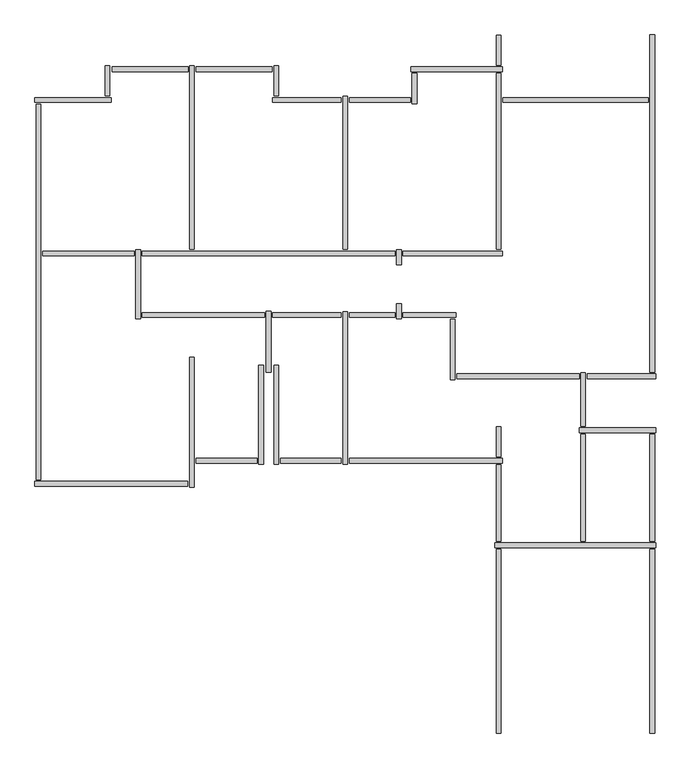
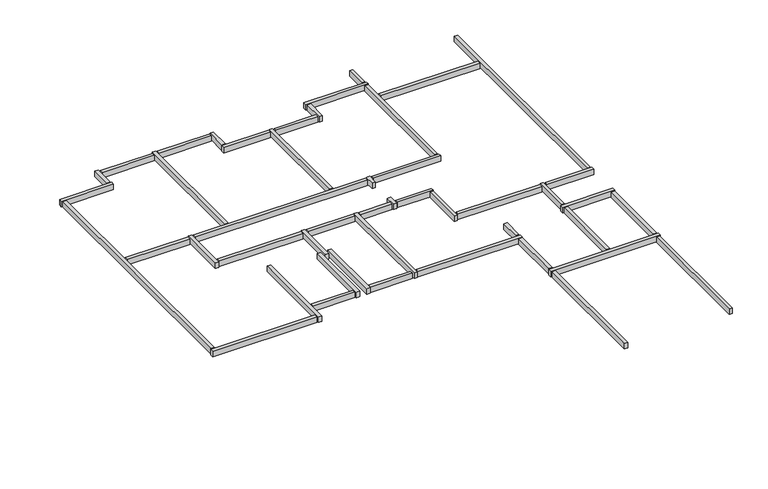
"""IFC4 building model written with IfcOpenShell, lengths in millimetres: beam geometry, Graute viga de respaldo3 : Graute viga de respaldo."""

from ifc_helpers import new_model, si_unit, frame, origin, place, context, project, spatial, polyline, outline, extrude, source, transform, mapped, element, save


def beam_e1de4ace(model_context):
    return source(origin(), model_context, "Body", "SweptSolid", [
        extrude(outline(polyline([(-70718.7587292, 62785.4278788), (-70624.7587292, 62785.4278788), (-70624.7587292, 59195.4278788), (-70718.7587292, 59195.4278788), (-70718.7587292, 62785.4278788)])), frame((0.0, 0.0, 2632.9999999), z_axis=(0.0, 0.0, 1.0), x_axis=(1.0, 0.0, 0.0)), (0.0, 0.0, 1.0), 167.0),
        extrude(outline(polyline([(-67718.7587292, 62785.4278788), (-67624.7587292, 62785.4278788), (-67624.7587292, 59195.4278788), (-67718.7587292, 59195.4278788), (-67718.7587292, 62785.4278788)])), frame((0.0, 0.0, 2632.9999999), z_axis=(0.0, 0.0, 1.0), x_axis=(1.0, 0.0, 0.0)), (0.0, 0.0, 1.0), 167.0),
        extrude(outline(polyline([(-75401.7587292, 64562.4278788), (-75401.7587292, 64468.4278788), (-76591.7587292, 64468.4278788), (-76591.7587292, 64562.4278788), (-75401.7587292, 64562.4278788)])), frame((0.0, 0.0, 2632.9999999), z_axis=(0.0, 0.0, 1.0), x_axis=(1.0, 0.0, 0.0)), (0.0, 0.0, 1.0), 167.0),
        extrude(outline(polyline([(-73751.7587292, 64562.4278788), (-73751.7587292, 64468.4278788), (-74941.7587292, 64468.4278788), (-74941.7587292, 64562.4278788), (-73751.7587292, 64562.4278788)])), frame((0.0, 0.0, 2632.9999999), z_axis=(0.0, 0.0, 1.0), x_axis=(1.0, 0.0, 0.0)), (0.0, 0.0, 1.0), 167.0),
        extrude(outline(polyline([(-77801.7587292, 68612.4278788), (-77801.7587292, 68518.4278788), (-79591.7587292, 68518.4278788), (-79591.7587292, 68612.4278788), (-77801.7587292, 68612.4278788)])), frame((0.0, 0.0, 2632.9999999), z_axis=(0.0, 0.0, 1.0), x_axis=(1.0, 0.0, 0.0)), (0.0, 0.0, 1.0), 167.0),
        extrude(outline(polyline([(-72401.7587292, 71612.4278788), (-72401.7587292, 71518.4278788), (-73591.7587292, 71518.4278788), (-73591.7587292, 71612.4278788), (-72401.7587292, 71612.4278788)])), frame((0.0, 0.0, 2632.9999999), z_axis=(0.0, 0.0, 1.0), x_axis=(1.0, 0.0, 0.0)), (0.0, 0.0, 1.0), 167.0),
        extrude(outline(polyline([(-72274.7587292, 71495.4278788), (-72368.7587292, 71495.4278788), (-72368.7587292, 72085.4278788), (-72274.7587292, 72085.4278788), (-72274.7587292, 71495.4278788)])), frame((0.0, 0.0, 2632.9999999), z_axis=(0.0, 0.0, 1.0), x_axis=(1.0, 0.0, 0.0)), (0.0, 0.0, 1.0), 167.0),
        extrude(outline(polyline([(-70601.7587292, 72212.4278788), (-70601.7587292, 72118.4278788), (-72391.7587292, 72118.4278788), (-72391.7587292, 72212.4278788), (-70601.7587292, 72212.4278788)])), frame((0.0, 0.0, 2632.9999999), z_axis=(0.0, 0.0, 1.0), x_axis=(1.0, 0.0, 0.0)), (0.0, 0.0, 1.0), 167.0),
        extrude(outline(polyline([(-72668.7587292, 68635.4278788), (-72574.7587292, 68635.4278788), (-72574.7587292, 68345.4278788), (-72668.7587292, 68345.4278788), (-72668.7587292, 68635.4278788)])), frame((0.0, 0.0, 2632.9999999), z_axis=(0.0, 0.0, 1.0), x_axis=(1.0, 0.0, 0.0)), (0.0, 0.0, 1.0), 167.0),
        extrude(outline(polyline([(-75251.7587292, 67412.4278788), (-75251.7587292, 67318.4278788), (-77641.7587292, 67318.4278788), (-77641.7587292, 67412.4278788), (-75251.7587292, 67412.4278788)])), frame((0.0, 0.0, 2632.9999999), z_axis=(0.0, 0.0, 1.0), x_axis=(1.0, 0.0, 0.0)), (0.0, 0.0, 1.0), 167.0),
        extrude(outline(polyline([(-73751.7587292, 67412.4278788), (-73751.7587292, 67318.4278788), (-75091.7587292, 67318.4278788), (-75091.7587292, 67412.4278788), (-73751.7587292, 67412.4278788)])), frame((0.0, 0.0, 2632.9999999), z_axis=(0.0, 0.0, 1.0), x_axis=(1.0, 0.0, 0.0)), (0.0, 0.0, 1.0), 167.0),
        extrude(outline(polyline([(-72701.7587292, 67412.4278788), (-72701.7587292, 67318.4278788), (-73591.7587292, 67318.4278788), (-73591.7587292, 67412.4278788), (-72701.7587292, 67412.4278788)])), frame((0.0, 0.0, 2632.9999999), z_axis=(0.0, 0.0, 1.0), x_axis=(1.0, 0.0, 0.0)), (0.0, 0.0, 1.0), 167.0),
        extrude(outline(polyline([(-72668.7587292, 67585.4278788), (-72574.7587292, 67585.4278788), (-72574.7587292, 67295.4278788), (-72668.7587292, 67295.4278788), (-72668.7587292, 67585.4278788)])), frame((0.0, 0.0, 2632.9999999), z_axis=(0.0, 0.0, 1.0), x_axis=(1.0, 0.0, 0.0)), (0.0, 0.0, 1.0), 167.0),
        extrude(outline(polyline([(-71511.7587292, 67412.4278788), (-71511.7587292, 67318.4278788), (-72541.7587292, 67318.4278788), (-72541.7587292, 67412.4278788), (-71511.7587292, 67412.4278788)])), frame((0.0, 0.0, 2632.9999999), z_axis=(0.0, 0.0, 1.0), x_axis=(1.0, 0.0, 0.0)), (0.0, 0.0, 1.0), 167.0),
        extrude(outline(polyline([(-71524.7587292, 66095.4278788), (-71618.7587292, 66095.4278788), (-71618.7587292, 67285.4278788), (-71524.7587292, 67285.4278788), (-71524.7587292, 66095.4278788)])), frame((0.0, 0.0, 2632.9999999), z_axis=(0.0, 0.0, 1.0), x_axis=(1.0, 0.0, 0.0)), (0.0, 0.0, 1.0), 167.0),
        extrude(outline(polyline([(-69091.7587292, 66212.4278788), (-69091.7587292, 66118.4278788), (-71491.7587292, 66118.4278788), (-71491.7587292, 66212.4278788), (-69091.7587292, 66212.4278788)])), frame((0.0, 0.0, 2632.9999999), z_axis=(0.0, 0.0, 1.0), x_axis=(1.0, 0.0, 0.0)), (0.0, 0.0, 1.0), 167.0),
        extrude(outline(polyline([(-73718.7587292, 67430.4278788), (-73624.7587292, 67430.4278788), (-73624.7587292, 64445.4278788), (-73718.7587292, 64445.4278788), (-73718.7587292, 67430.4278788)])), frame((0.0, 0.0, 2632.9999999), z_axis=(0.0, 0.0, 1.0), x_axis=(1.0, 0.0, 0.0)), (0.0, 0.0, 1.0), 167.0),
        extrude(outline(polyline([(-70601.7587292, 64562.4278788), (-70601.7587292, 64468.4278788), (-73591.7587292, 64468.4278788), (-73591.7587292, 64562.4278788), (-70601.7587292, 64562.4278788)])), frame((0.0, 0.0, 2632.9999999), z_axis=(0.0, 0.0, 1.0), x_axis=(1.0, 0.0, 0.0)), (0.0, 0.0, 1.0), 167.0),
        extrude(outline(polyline([(-70718.7587292, 65185.4278788), (-70624.7587292, 65185.4278788), (-70624.7587292, 64595.4278788), (-70718.7587292, 64595.4278788), (-70718.7587292, 65185.4278788)])), frame((0.0, 0.0, 2632.9999999), z_axis=(0.0, 0.0, 1.0), x_axis=(1.0, 0.0, 0.0)), (0.0, 0.0, 1.0), 167.0),
        extrude(outline(polyline([(-70624.7587292, 62945.4278788), (-70718.7587292, 62945.4278788), (-70718.7587292, 64435.4278788), (-70624.7587292, 64435.4278788), (-70624.7587292, 62945.4278788)])), frame((0.0, 0.0, 2632.9999999), z_axis=(0.0, 0.0, 1.0), x_axis=(1.0, 0.0, 0.0)), (0.0, 0.0, 1.0), 167.0),
        extrude(outline(polyline([(-67624.7587292, 62945.4278788), (-67718.7587292, 62945.4278788), (-67718.7587292, 65035.4278788), (-67624.7587292, 65035.4278788), (-67624.7587292, 62945.4278788)])), frame((0.0, 0.0, 2632.9999999), z_axis=(0.0, 0.0, 1.0), x_axis=(1.0, 0.0, 0.0)), (0.0, 0.0, 1.0), 167.0),
        extrude(outline(polyline([(-68974.7587292, 62945.4278788), (-69068.7587292, 62945.4278788), (-69068.7587292, 65035.4278788), (-68974.7587292, 65035.4278788), (-68974.7587292, 62945.4278788)])), frame((0.0, 0.0, 2632.9999999), z_axis=(0.0, 0.0, 1.0), x_axis=(1.0, 0.0, 0.0)), (0.0, 0.0, 1.0), 167.0),
        extrude(outline(polyline([(-69068.7587292, 66235.4278788), (-68974.7587292, 66235.4278788), (-68974.7587292, 65195.4278788), (-69068.7587292, 65195.4278788), (-69068.7587292, 66235.4278788)])), frame((0.0, 0.0, 2632.9999999), z_axis=(0.0, 0.0, 1.0), x_axis=(1.0, 0.0, 0.0)), (0.0, 0.0, 1.0), 167.0),
        extrude(outline(polyline([(-67751.7587292, 71612.4278788), (-67751.7587292, 71518.4278788), (-70591.7587292, 71518.4278788), (-70591.7587292, 71612.4278788), (-67751.7587292, 71612.4278788)])), frame((0.0, 0.0, 2632.9999999), z_axis=(0.0, 0.0, 1.0), x_axis=(1.0, 0.0, 0.0)), (0.0, 0.0, 1.0), 167.0),
        extrude(outline(polyline([(-70624.7587292, 68645.4278788), (-70718.7587292, 68645.4278788), (-70718.7587292, 72085.4278788), (-70624.7587292, 72085.4278788), (-70624.7587292, 68645.4278788)])), frame((0.0, 0.0, 2632.9999999), z_axis=(0.0, 0.0, 1.0), x_axis=(1.0, 0.0, 0.0)), (0.0, 0.0, 1.0), 167.0),
        extrude(outline(polyline([(-70601.7587292, 68612.4278788), (-70601.7587292, 68518.4278788), (-72541.7587292, 68518.4278788), (-72541.7587292, 68612.4278788), (-70601.7587292, 68612.4278788)])), frame((0.0, 0.0, 2632.9999999), z_axis=(0.0, 0.0, 1.0), x_axis=(1.0, 0.0, 0.0)), (0.0, 0.0, 1.0), 167.0),
        extrude(outline(polyline([(-72701.7587292, 68612.4278788), (-72701.7587292, 68518.4278788), (-77641.7587292, 68518.4278788), (-77641.7587292, 68612.4278788), (-72701.7587292, 68612.4278788)])), frame((0.0, 0.0, 2632.9999999), z_axis=(0.0, 0.0, 1.0), x_axis=(1.0, 0.0, 0.0)), (0.0, 0.0, 1.0), 167.0),
        extrude(outline(polyline([(-73718.7587292, 71635.4278788), (-73624.7587292, 71635.4278788), (-73624.7587292, 68645.4278788), (-73718.7587292, 68645.4278788), (-73718.7587292, 71635.4278788)])), frame((0.0, 0.0, 2632.9999999), z_axis=(0.0, 0.0, 1.0), x_axis=(1.0, 0.0, 0.0)), (0.0, 0.0, 1.0), 167.0),
        extrude(outline(polyline([(-75091.7587292, 71518.4278788), (-75091.7587292, 71612.4278788), (-73751.7587292, 71612.4278788), (-73751.7587292, 71518.4278788), (-75091.7587292, 71518.4278788)])), frame((0.0, 0.0, 2632.9999999), z_axis=(0.0, 0.0, 1.0), x_axis=(1.0, 0.0, 0.0)), (0.0, 0.0, 1.0), 167.0),
        extrude(outline(polyline([(-75068.7587292, 72235.4278788), (-74974.7587292, 72235.4278788), (-74974.7587292, 71645.4278788), (-75068.7587292, 71645.4278788), (-75068.7587292, 72235.4278788)])), frame((0.0, 0.0, 2632.9999999), z_axis=(0.0, 0.0, 1.0), x_axis=(1.0, 0.0, 0.0)), (0.0, 0.0, 1.0), 167.0),
        extrude(outline(polyline([(-75101.7587292, 72212.4278788), (-75101.7587292, 72118.4278788), (-76591.7587292, 72118.4278788), (-76591.7587292, 72212.4278788), (-75101.7587292, 72212.4278788)])), frame((0.0, 0.0, 2632.9999999), z_axis=(0.0, 0.0, 1.0), x_axis=(1.0, 0.0, 0.0)), (0.0, 0.0, 1.0), 167.0),
        extrude(outline(polyline([(-78230.736554, 72117.4278788), (-78230.736554, 72212.4278788), (-76741.7587292, 72212.4278788), (-76741.7587292, 72117.4278788), (-78230.736554, 72117.4278788)])), frame((0.0, 0.0, 2617.1856208), z_axis=(0.0, 0.0, 1.0), x_axis=(1.0, 0.0, 0.0)), (0.0, 0.0, 1.0), 165.0),
        extrude(outline(polyline([(-79624.7587292, 64145.4278788), (-79718.7587292, 64145.4278788), (-79718.7587292, 71485.4278788), (-79624.7587292, 71485.4278788), (-79624.7587292, 64145.4278788)])), frame((0.0, 0.0, 2632.9999999), z_axis=(0.0, 0.0, 1.0), x_axis=(1.0, 0.0, 0.0)), (0.0, 0.0, 1.0), 167.0),
        extrude(outline(polyline([(-77674.7587292, 67295.4278788), (-77768.7587292, 67295.4278788), (-77768.7587292, 68640.7810915), (-77674.7587292, 68640.7810915), (-77674.7587292, 67295.4278788)])), frame((0.0, 0.0, 2632.9999999), z_axis=(0.0, 0.0, 1.0), x_axis=(1.0, 0.0, 0.0)), (0.0, 0.0, 1.0), 167.0),
        extrude(outline(polyline([(-75124.7587292, 66245.4278788), (-75218.7587292, 66245.4278788), (-75218.7587292, 67435.4278788), (-75124.7587292, 67435.4278788), (-75124.7587292, 66245.4278788)])), frame((0.0, 0.0, 2632.9999999), z_axis=(0.0, 0.0, 1.0), x_axis=(1.0, 0.0, 0.0)), (0.0, 0.0, 1.0), 167.0),
        extrude(outline(polyline([(-75274.7587292, 64445.4278788), (-75368.7587292, 64445.4278788), (-75368.7587292, 66385.4278788), (-75274.7587292, 66385.4278788), (-75274.7587292, 64445.4278788)])), frame((0.0, 0.0, 2632.9999999), z_axis=(0.0, 0.0, 1.0), x_axis=(1.0, 0.0, 0.0)), (0.0, 0.0, 1.0), 167.0),
        extrude(outline(polyline([(-74974.7587292, 64445.4278788), (-75068.7587292, 64445.4278788), (-75068.7587292, 66385.4278788), (-74974.7587292, 66385.4278788), (-74974.7587292, 64445.4278788)])), frame((0.0, 0.0, 2632.9999999), z_axis=(0.0, 0.0, 1.0), x_axis=(1.0, 0.0, 0.0)), (0.0, 0.0, 1.0), 167.0),
        extrude(outline(polyline([(-76624.7587292, 63995.4278788), (-76718.7587292, 63995.4278788), (-76718.7587292, 66535.4278788), (-76624.7587292, 66535.4278788), (-76624.7587292, 63995.4278788)])), frame((0.0, 0.0, 2632.9999999), z_axis=(0.0, 0.0, 1.0), x_axis=(1.0, 0.0, 0.0)), (0.0, 0.0, 1.0), 167.0),
        extrude(outline(polyline([(-79741.7587292, 64018.4278788), (-79741.7587292, 64112.4278788), (-76751.7587292, 64112.4278788), (-76751.7587292, 64018.4278788), (-79741.7587292, 64018.4278788)])), frame((0.0, 0.0, 2632.9999999), z_axis=(0.0, 0.0, 1.0), x_axis=(1.0, 0.0, 0.0)), (0.0, 0.0, 1.0), 167.0),
        extrude(outline(polyline([(-78368.7587292, 72235.4278788), (-78274.7587292, 72235.4278788), (-78274.7587292, 71645.4278788), (-78368.7587292, 71645.4278788), (-78368.7587292, 72235.4278788)])), frame((0.0, 0.0, 2632.9999999), z_axis=(0.0, 0.0, 1.0), x_axis=(1.0, 0.0, 0.0)), (0.0, 0.0, 1.0), 167.0),
        extrude(outline(polyline([(-78251.7587292, 71612.4278788), (-78251.7587292, 71518.4278788), (-79741.7587292, 71518.4278788), (-79741.7587292, 71612.4278788), (-78251.7587292, 71612.4278788)])), frame((0.0, 0.0, 2632.9999999), z_axis=(0.0, 0.0, 1.0), x_axis=(1.0, 0.0, 0.0)), (0.0, 0.0, 1.0), 167.0),
        extrude(outline(polyline([(-76718.7587292, 72235.4278788), (-76624.7587292, 72235.4278788), (-76624.7587292, 68645.4278788), (-76718.7587292, 68645.4278788), (-76718.7587292, 72235.4278788)])), frame((0.0, 0.0, 2632.9999999), z_axis=(0.0, 0.0, 1.0), x_axis=(1.0, 0.0, 0.0)), (0.0, 0.0, 1.0), 167.0),
        extrude(outline(polyline([(-70718.7587292, 72835.4278788), (-70624.7587292, 72835.4278788), (-70624.7587292, 72245.4278788), (-70718.7587292, 72245.4278788), (-70718.7587292, 72835.4278788)])), frame((0.0, 0.0, 2632.9999999), z_axis=(0.0, 0.0, 1.0), x_axis=(1.0, 0.0, 0.0)), (0.0, 0.0, 1.0), 167.0),
        extrude(outline(polyline([(-67601.7587292, 65162.4278788), (-67601.7587292, 65068.4278788), (-69091.7587292, 65068.4278788), (-69091.7587292, 65162.4278788), (-67601.7587292, 65162.4278788)])), frame((0.0, 0.0, 2632.9999999), z_axis=(0.0, 0.0, 1.0), x_axis=(1.0, 0.0, 0.0)), (0.0, 0.0, 1.0), 167.0),
        extrude(outline(polyline([(-67601.7587292, 62912.4278788), (-67601.7587292, 62818.4278788), (-70741.7587292, 62818.4278788), (-70741.7587292, 62912.4278788), (-67601.7587292, 62912.4278788)])), frame((0.0, 0.0, 2632.9999999), z_axis=(0.0, 0.0, 1.0), x_axis=(1.0, 0.0, 0.0)), (0.0, 0.0, 1.0), 167.0),
        extrude(outline(polyline([(-67601.7587292, 66212.4278788), (-67601.7587292, 66118.4278788), (-68941.7587292, 66118.4278788), (-68941.7587292, 66212.4278788), (-67601.7587292, 66212.4278788)])), frame((0.0, 0.0, 2632.9999999), z_axis=(0.0, 0.0, 1.0), x_axis=(1.0, 0.0, 0.0)), (0.0, 0.0, 1.0), 167.0),
        extrude(outline(polyline([(-67718.7587292, 72837.9577736), (-67624.7587292, 72837.9577736), (-67624.7587292, 66245.4278788), (-67718.7587292, 66245.4278788), (-67718.7587292, 72837.9577736)])), frame((0.0, 0.0, 2632.9999999), z_axis=(0.0, 0.0, 1.0), x_axis=(1.0, 0.0, 0.0)), (0.0, 0.0, 1.0), 167.0),
    ])


if __name__ == "__main__":
    model = new_model("IFC4")
    model_context = context("Model", 3, world=origin())
    ifc_project = project(units=[si_unit("LENGTHUNIT", "METRE", prefix="MILLI")], contexts=[model_context])
    site = spatial("IfcSite", under=ifc_project)
    building = spatial("IfcBuilding", under=site)
    placement = place(None, origin())
    beam_shape = beam_e1de4ace(model_context)
    element("IfcBeam", 1, ObjectType="Graute viga de respaldo3 : Graute viga de respaldo", at=placement, inside=building, context=model_context, shape_type="MappedRepresentation", body=[
        mapped(beam_shape, transform((0.0, 0.0, 0.0), x_axis=(1.0, 0.0, 0.0), y_axis=(0.0, 1.0, 0.0), z_axis=(0.0, 0.0, 1.0))),
    ])
    save(model, "model.ifc")

# Revit data of these elements
# Element 1 (IfcBeam, "Graute viga de respaldo3 : Graute viga de respaldo")
#   Materials on its faces: "Concreto, Faixa de areia/cimento"
# Materials
#   "Concreto, Faixa de areia/cimento": class "Concreto", colour RGB 127 127 127, transparency 0, Description = "Revestimento de laje de concreto", Cost = 0
